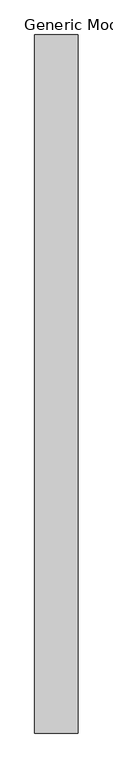
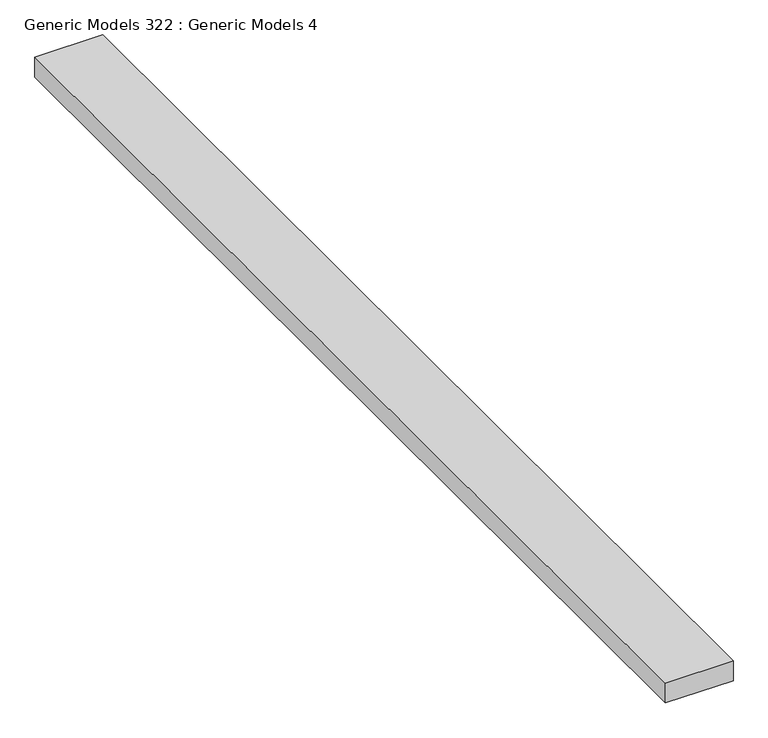
"""IFC4 building model written with IfcOpenShell, lengths in millimetres: proxy geometry, Generic Models 322 : Generic Models 4."""

from ifc_helpers import new_model, si_unit, frame, origin, place, context, project, spatial, polyline, outline, extrude, source, transform, mapped, element, save


def generic_models_322_generic_models_4_90198746(model_context):
    return source(origin(), model_context, "Body", "SweptSolid", [
        extrude(outline(polyline([(-5937.4236296, -5493.3230338), (-6426.3736296, -5493.3230338), (-6426.3736296, 2393.3769662), (-5937.4236296, 2393.3769662), (-5937.4236296, -5493.3230338)])), frame((0.0, 0.0, 122802.396), z_axis=(0.0, 0.0, 1.0), x_axis=(1.0, 0.0, 0.0)), (0.0, 0.0, 1.0), 150.8125),
    ])


if __name__ == "__main__":
    model = new_model("IFC4")
    model_context = context("Model", 3, world=origin())
    ifc_project = project(units=[si_unit("LENGTHUNIT", "METRE", prefix="MILLI")], contexts=[model_context])
    site = spatial("IfcSite", under=ifc_project)
    building = spatial("IfcBuilding", under=site)
    placement = place(None, origin())
    generic_models_322_generic_models_4_shape = generic_models_322_generic_models_4_90198746(model_context)
    element("IfcBuildingElementProxy", 1, Name="Generic Models 322 : Generic Models 4", ObjectType="Generic Models 322 : Generic Models 4", at=placement, inside=building, context=model_context, shape_type="MappedRepresentation", body=[
        mapped(generic_models_322_generic_models_4_shape, transform((0.0, 0.0, 0.0), x_axis=(1.0, 0.0, 0.0), y_axis=(0.0, 1.0, 0.0), z_axis=(0.0, 0.0, 1.0))),
    ])
    save(model, "model.ifc")

# Revit data of these elements
# Element 1 (IfcBuildingElementProxy, "Generic Models 322 : Generic Models 4")
#   Materials on its faces: "_COMPACTED GRADE"
# Materials
#   "_COMPACTED GRADE": class "Generic", colour RGB 120 100 58, transparency 0, Cost = 0
